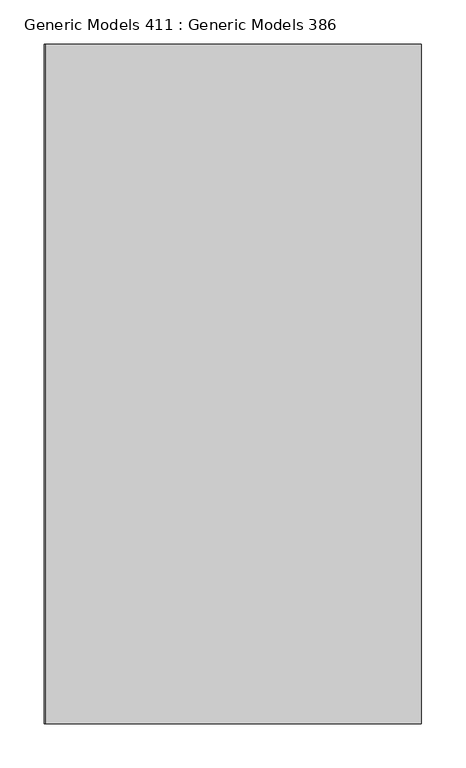
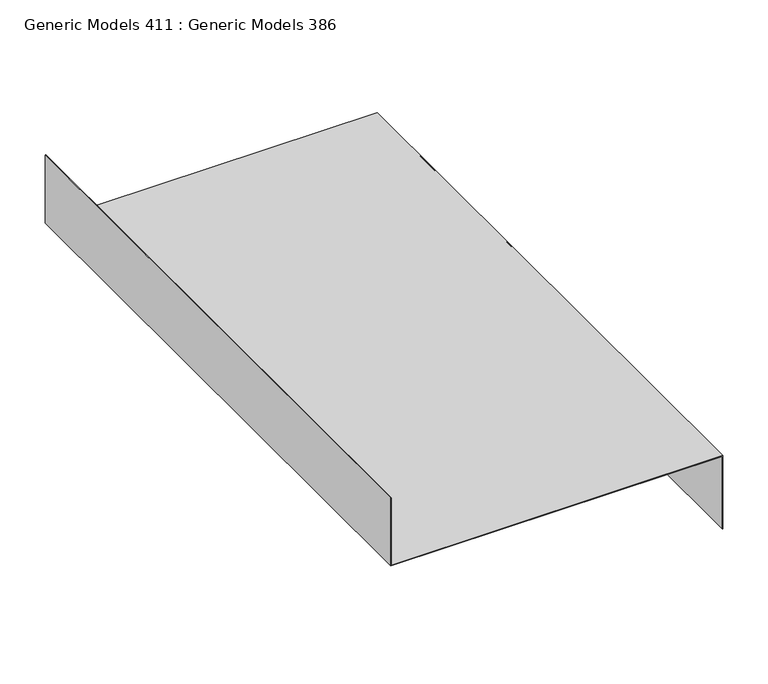
"""IFC4 building model written with IfcOpenShell, lengths in millimetres: proxy geometry, Generic Models 411 : Generic Models 386."""

import ifcopenshell
import ifcopenshell.guid

model = None  # the IFC model being written
_history = None  # IfcOwnerHistory: only IFC2X3 demands one
_inside = {}  # id of a spatial element -> (the spatial element, [elements in it])
_under = {}  # id of a project, library or spatial element -> (it, [spatial elements below it])
_declared = {}  # id of a project -> (the project, [libraries it declares])
_typed = {}  # id of a type object -> (the type object, [elements of that type])
_made_of = {}  # id of a material, layer set ... -> (it, [elements and type objects made of it])


def new_model(schema):
    """Start an empty IFC model of exactly this schema.

    Asked for "IFC4X3", IfcOpenShell would pick the latest addendum, in which some entities
    have other attributes; the version numbers below select the first issue.
    IFC2X3 requires an IfcOwnerHistory on every rooted entity: one is made here for all.
    """
    global model, _history
    if schema == "IFC4X3":
        model = ifcopenshell.file(schema_version=(4, 3, 0, 0))
    else:
        model = ifcopenshell.file(schema=schema)
    _inside.clear()
    _under.clear()
    _declared.clear()
    _typed.clear()
    _made_of.clear()
    _history = None
    if model.schema == "IFC2X3":
        org = make("IfcOrganization", Name="unknown")
        user = make(
            "IfcPersonAndOrganization",
            ThePerson=make("IfcPerson", FamilyName="unknown"),
            TheOrganization=org,
        )
        app = make(
            "IfcApplication",
            ApplicationDeveloper=org,
            Version="unknown",
            ApplicationFullName="unknown",
            ApplicationIdentifier="unknown",
        )
        _history = make(
            "IfcOwnerHistory",
            OwningUser=user,
            OwningApplication=app,
            ChangeAction="ADDED",
            CreationDate=0,
        )
    return model


def make(cls, **values):
    """One entity of the class cls with the attributes given. An attribute that is None is left unset."""
    return model.create_entity(
        cls, **{name: value for name, value in values.items() if value is not None}
    )


def rooted(cls, **values):
    """An entity with a GlobalId (a new one), such as an element, a storey or a relation."""
    return make(cls, GlobalId=ifcopenshell.guid.new(), OwnerHistory=_history, **values)


def si_unit(unit_type, name, prefix=None):
    """IfcSIUnit, for example si_unit("LENGTHUNIT", "METRE", prefix="MILLI")."""
    return make("IfcSIUnit", UnitType=unit_type, Prefix=prefix, Name=name)


def assignment(units):
    """IfcUnitAssignment: the units of a project."""
    return None if units is None else make("IfcUnitAssignment", Units=units)


def point(xyz):
    """IfcCartesianPoint."""
    return None if xyz is None else make("IfcCartesianPoint", Coordinates=xyz)


def direction(xyz):
    """IfcDirection."""
    return None if xyz is None else make("IfcDirection", DirectionRatios=xyz)


def frame(location, z_axis=None, x_axis=None):
    """IfcAxis2Placement3D, a coordinate frame: its origin and axes. An axis left out is left unset."""
    return make(
        "IfcAxis2Placement3D",
        Location=point(location),
        Axis=direction(z_axis),
        RefDirection=direction(x_axis),
    )


def origin():
    """The frame at (0, 0, 0) with its axes left unset."""
    return frame((0.0, 0.0, 0.0))


def place(relative_to, where):
    """IfcLocalPlacement: puts the frame where relative to a parent placement (None: the world)."""
    return make(
        "IfcLocalPlacement", PlacementRelTo=relative_to, RelativePlacement=where
    )


def context(
    kind, dimensions, precision=None, world=None, true_north=None, identifier=None
):
    """IfcGeometricRepresentationContext, for example the 3D "Model" context."""
    return make(
        "IfcGeometricRepresentationContext",
        ContextIdentifier=identifier,
        ContextType=kind,
        CoordinateSpaceDimension=dimensions,
        Precision=precision,
        WorldCoordinateSystem=world,
        TrueNorth=true_north,
    )


def project(units=None, contexts=None):
    """IfcProject with its units and contexts."""
    return rooted(
        "IfcProject",
        Name="project",
        RepresentationContexts=contexts,
        UnitsInContext=assignment(units),
    )


def spatial(cls, under=None, at=None, **own):
    """A site, building, storey or space (cls), placed at a placement, below another one or the project."""
    s = rooted(cls, ObjectPlacement=at, **own)
    if under is not None:
        _under.setdefault(under.id(), (under, []))[1].append(s)
    return s


def polyline(points):
    """IfcPolyline through the points."""
    return make("IfcPolyline", Points=[point(p) for p in points])


def outline(outer, holes=None, kind="AREA"):
    """IfcArbitraryClosedProfileDef: a profile drawn as a closed curve; with holes, ...WithVoids."""
    if holes is None:
        return make("IfcArbitraryClosedProfileDef", ProfileType=kind, OuterCurve=outer)
    return make(
        "IfcArbitraryProfileDefWithVoids",
        ProfileType=kind,
        OuterCurve=outer,
        InnerCurves=holes,
    )


def extrude(swept, where, along, depth):
    """IfcExtrudedAreaSolid: the profile swept, set in the frame where, extruded along a direction by depth."""
    return make(
        "IfcExtrudedAreaSolid",
        SweptArea=swept,
        Position=where,
        ExtrudedDirection=direction(along),
        Depth=depth,
    )


def shape(context_of_items, identifier, shape_type, items):
    """IfcShapeRepresentation: the items that make up one representation, for example the "Body"."""
    return make(
        "IfcShapeRepresentation",
        ContextOfItems=context_of_items,
        RepresentationIdentifier=identifier,
        RepresentationType=shape_type,
        Items=items,
    )


def source(mapping_origin, context_of_items, identifier, shape_type, items):
    """IfcRepresentationMap: a shape defined once, which mapped items show again and again."""
    return make(
        "IfcRepresentationMap",
        MappingOrigin=mapping_origin,
        MappedRepresentation=shape(context_of_items, identifier, shape_type, items),
    )


def transform(
    local_origin,
    x_axis=None,
    y_axis=None,
    z_axis=None,
    scale=None,
    scale2=None,
    scale3=None,
    uniform=True,
):
    """IfcCartesianTransformationOperator3D, or its non-uniform kind. x_axis, y_axis, z_axis: its Axis1, 2, 3."""
    if uniform:
        return make(
            "IfcCartesianTransformationOperator3D",
            Axis1=direction(x_axis),
            Axis2=direction(y_axis),
            LocalOrigin=point(local_origin),
            Scale=scale,
            Axis3=direction(z_axis),
        )
    return make(
        "IfcCartesianTransformationOperator3DnonUniform",
        Axis1=direction(x_axis),
        Axis2=direction(y_axis),
        LocalOrigin=point(local_origin),
        Scale=scale,
        Axis3=direction(z_axis),
        Scale2=scale2,
        Scale3=scale3,
    )


def mapped(mapping_source, mapping_target):
    """IfcMappedItem: shows the shape of a source again, moved by a transform."""
    return make(
        "IfcMappedItem", MappingSource=mapping_source, MappingTarget=mapping_target
    )


def made_of(thing, what):
    """Note that an element or type object is made of a material, layer set ...; save() writes the relation."""
    if what is not None:
        _made_of.setdefault(what.id(), (what, []))[1].append(thing)
    return thing


def element(
    cls,
    number,
    at=None,
    inside=None,
    cuts=None,
    type_object=None,
    material=None,
    context=None,
    identifier="Body",
    shape_type=None,
    held_by="IfcProductDefinitionShape",
    body=None,
    shapes=None,
    **own,
):
    """One element of the class cls, such as IfcWall. Its Tag is "e" and its number.

    at: its placement. inside: the storey or other place that contains it. cuts: it is an
    opening in that element (IfcRelVoidsElement). A single representation is given by context,
    identifier, shape_type and body (its items); several are given by shapes. held_by: the class
    of the entity that holds the representations. save() writes the other relations.
    """
    e = rooted(cls, Tag="e%d" % number, ObjectPlacement=at, **own)
    if body is not None:
        shapes = [shape(context, identifier, shape_type, body)]
    if shapes is not None:
        e.Representation = make(held_by, Representations=shapes)
    if inside is not None:
        _inside.setdefault(inside.id(), (inside, []))[1].append(e)
    if cuts is not None:
        rooted(
            "IfcRelVoidsElement", RelatingBuildingElement=cuts, RelatedOpeningElement=e
        )
    if type_object is not None:
        _typed.setdefault(type_object.id(), (type_object, []))[1].append(e)
    return made_of(e, material)


def aggregate(whole, parts):
    """IfcRelAggregates: a whole, such as a stair, and the parts it consists of."""
    return rooted("IfcRelAggregates", RelatingObject=whole, RelatedObjects=parts)


def save(model, path):
    """Write the relations noted so far, then the file.

    IfcRelAggregates (storeys below a building ...), IfcRelContainedInSpatialStructure (elements
    in a storey), IfcRelDefinesByType, IfcRelAssociatesMaterial and IfcRelDeclares: one each for
    every whole, place, type object, material and project.
    """
    for whole, parts in _under.values():
        aggregate(whole, parts)
    for where, things in _inside.values():
        rooted(
            "IfcRelContainedInSpatialStructure",
            RelatedElements=things,
            RelatingStructure=where,
        )
    for kind, things in _typed.values():
        rooted("IfcRelDefinesByType", RelatedObjects=things, RelatingType=kind)
    for what, things in _made_of.values():
        rooted("IfcRelAssociatesMaterial", RelatedObjects=things, RelatingMaterial=what)
    for by, libraries in _declared.values():
        rooted("IfcRelDeclares", RelatingContext=by, RelatedDefinitions=libraries)
    model.write(path)


def generic_models_411_generic_models_386_1a9935e2(model_context):
    return source(origin(), model_context, "Body", "SweptSolid", [
        extrude(outline(polyline([(127251.4917289, -6626.6337799), (127153.4757007, -6626.6337799), (127153.4757007, -6625.8400299), (127252.2854789, -6625.8400299), (127252.2854789, -7048.7579637), (127343.1367561, -7048.7579637), (127343.1367561, -7049.5517137), (127251.4917289, -7049.5517137), (127251.4917289, -6626.6337799)])), frame((0.0, -4250.542257, 0.0), z_axis=(0.0, 1.0, 0.0), x_axis=(0.0, 0.0, 1.0)), (0.0, 0.0, 1.0), 763.8192232),
    ])


if __name__ == "__main__":
    model = new_model("IFC4")
    model_context = context("Model", 3, world=origin())
    ifc_project = project(units=[si_unit("LENGTHUNIT", "METRE", prefix="MILLI")], contexts=[model_context])
    site = spatial("IfcSite", under=ifc_project)
    building = spatial("IfcBuilding", under=site)
    placement = place(None, origin())
    generic_models_411_generic_models_386_shape = generic_models_411_generic_models_386_1a9935e2(model_context)
    element("IfcBuildingElementProxy", 1, Name="Generic Models 411 : Generic Models 386", ObjectType="Generic Models 411 : Generic Models 386", at=placement, inside=building, context=model_context, shape_type="MappedRepresentation", body=[
        mapped(generic_models_411_generic_models_386_shape, transform((0.0, 0.0, 0.0), x_axis=(1.0, 0.0, 0.0), y_axis=(0.0, 1.0, 0.0), z_axis=(0.0, 0.0, 1.0))),
    ])
    save(model, "model.ifc")

# Revit data of these elements
# Element 1 (IfcBuildingElementProxy, "Generic Models 411 : Generic Models 386")
#   Materials on its faces: "_(2) LAYERS NO. 30 ASTM D226 ASPHALT SATURATED ORGANIC FELT @ ROOF"
# Materials
#   "_(2) LAYERS NO. 30 ASTM D226 ASPHALT SATURATED ORGANIC FELT @ ROOF": class "Generic", colour RGB 67 154 161, transparency 0, Cost = 0
